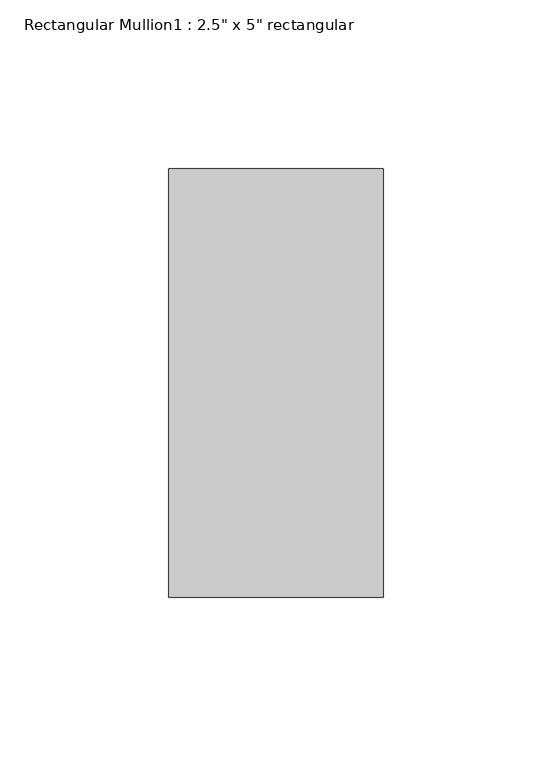
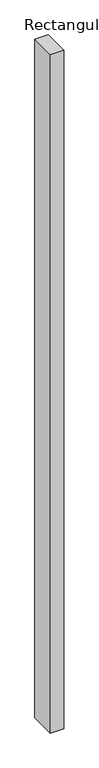
"""IFC4 building model written with IfcOpenShell, lengths in millimetres: member geometry."""

from ifc_helpers import new_model, si_unit, frame, origin, place, context, project, spatial, polyline, outline, extrude, source, transform, mapped, element, save


def member_7b18d258(model_context):
    return source(origin(), model_context, "Body", "SweptSolid", [
        extrude(outline(polyline([(31.75, 63.5), (31.75, -63.5), (-31.75, -63.5), (-31.75, 63.5), (31.75, 63.5)])), frame((0.0, 0.0, -3382.4333333), z_axis=(0.0, 0.0, 1.0), x_axis=(1.0, 0.0, 0.0)), (0.0, 0.0, 1.0), 3382.4333333),
    ])


if __name__ == "__main__":
    model = new_model("IFC4")
    model_context = context("Model", 3, world=origin())
    ifc_project = project(units=[si_unit("LENGTHUNIT", "METRE", prefix="MILLI")], contexts=[model_context])
    site = spatial("IfcSite", under=ifc_project)
    building = spatial("IfcBuilding", under=site)
    placement = place(None, origin())
    member_shape = member_7b18d258(model_context)
    element("IfcMember", 1, ObjectType="Rectangular Mullion1 : 2.5\" x 5\" rectangular", at=placement, inside=building, context=model_context, shape_type="MappedRepresentation", body=[
        mapped(member_shape, transform((0.0, 0.0, 0.0), x_axis=(1.0, 0.0, 0.0), y_axis=(0.0, 1.0, 0.0), z_axis=(0.0, 0.0, 1.0))),
    ])
    save(model, "model.ifc")

# Revit data of these elements
# Type "Rectangular Mullion1 : 2.5\" x 5\" rectangular"
#   built-in parameter 1007304 = 0.416667 (stored number, unit not read)
#   built-in parameter 1007301 = 0.104167 (stored number, unit not read)
#   built-in parameter 1007300 = 0.104167 (stored number, unit not read)
# Element 1 (IfcMember, "Rectangular Mullion1 : 2.5\" x 5\" rectangular")
#   Materials on its faces: "support-frame"
# Materials
#   "support-frame": class "Unassigned", colour RGB 233 233 233, transparency 0, Cost = 0
